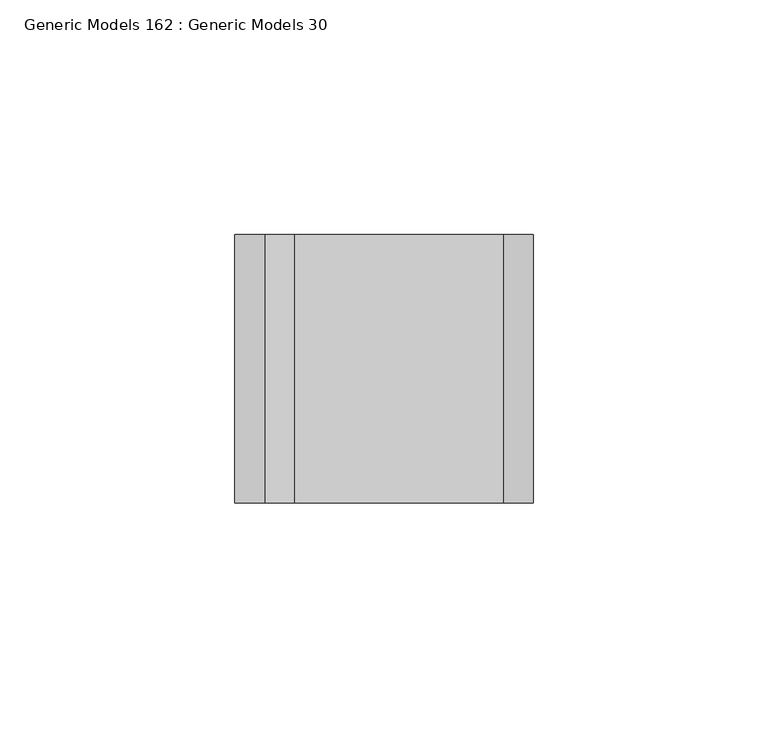
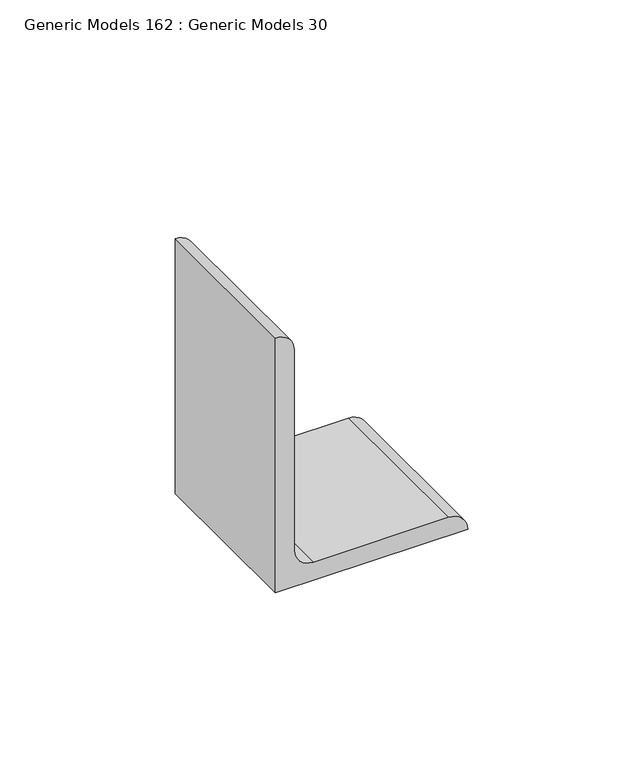
"""IFC4 building model written with IfcOpenShell, lengths in millimetres: proxy geometry, Generic Models 162 : Generic Models 30."""

from ifc_helpers import new_model, si_unit, point, frame, frame_2d, origin, place, context, project, spatial, polyline, circle_curve, trimmed, segment, composite_curve, outline, extrude, source, transform, mapped, element, save


def generic_models_162_generic_models_30_9cc2ba71(model_context):
    return source(origin(), model_context, "Body", "SweptSolid", [
        extrude(outline(composite_curve([segment(polyline([(266401.55, 34434.4590778), (266401.55, 34497.9590778)]), True, "CONTINUOUS"), segment(trimmed(circle_curve(frame_2d((266401.55, 34491.6090778)), 6.35), [point((266401.55, 34497.9590778))], [point((266407.9, 34491.6090778))], False, "CARTESIAN"), True, "CONTINUOUS"), segment(polyline([(266407.9, 34491.6090778), (266407.9, 34447.1590778)]), True, "CONTINUOUS"), segment(trimmed(circle_curve(frame_2d((266414.25, 34447.1590778)), 6.35), [point((266407.9, 34447.1590778))], [point((266414.25, 34440.8090778))], True, "CARTESIAN"), True, "CONTINUOUS"), segment(polyline([(266414.25, 34440.8090778), (266484.1, 34440.8090778)]), True, "CONTINUOUS"), segment(trimmed(circle_curve(frame_2d((266484.1, 34434.4590778)), 6.35), [point((266484.1, 34440.8090778))], [point((266490.45, 34434.4590778))], False, "CARTESIAN"), True, "CONTINUOUS"), segment(polyline([(266490.45, 34434.4590778), (266401.55, 34434.4590778)]), True, "CONTINUOUS")], self_intersect=False)), frame((0.0, 41007.6196612, 0.0), z_axis=(0.0, 1.0, 0.0), x_axis=(0.0, 0.0, 1.0)), (0.0, 0.0, 1.0), 57.15),
    ])


if __name__ == "__main__":
    model = new_model("IFC4")
    model_context = context("Model", 3, world=origin())
    ifc_project = project(units=[si_unit("LENGTHUNIT", "METRE", prefix="MILLI")], contexts=[model_context])
    site = spatial("IfcSite", under=ifc_project)
    building = spatial("IfcBuilding", under=site)
    placement = place(None, origin())
    generic_models_162_generic_models_30_shape = generic_models_162_generic_models_30_9cc2ba71(model_context)
    element("IfcBuildingElementProxy", 1, Name="Generic Models 162 : Generic Models 30", ObjectType="Generic Models 162 : Generic Models 30", at=placement, inside=building, context=model_context, shape_type="MappedRepresentation", body=[
        mapped(generic_models_162_generic_models_30_shape, transform((0.0, 0.0, 0.0), x_axis=(1.0, 0.0, 0.0), y_axis=(0.0, 1.0, 0.0), z_axis=(0.0, 0.0, 1.0))),
    ])
    save(model, "model.ifc")

# Revit data of these elements
# Element 1 (IfcBuildingElementProxy, "Generic Models 162 : Generic Models 30")
#   Materials on its faces: "GALV 3 1/2\"X 2 1/2\" X 1/4\" STEEL ANGLE - WELD TO VERTICAL STEEL ANGLE"
# Materials
#   "GALV 3 1/2\"X 2 1/2\" X 1/4\" STEEL ANGLE - WELD TO VERTICAL STEEL ANGLE": class "Metal", colour RGB 199 199 199, transparency 0, Description = "Structural steel, ASTM A36 Grade B, mill finish", Cost = 0
